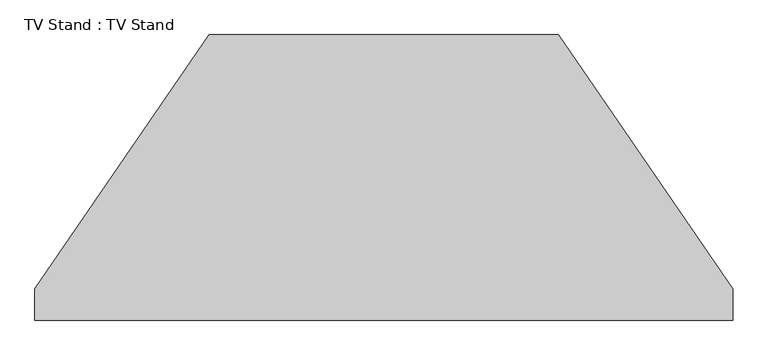
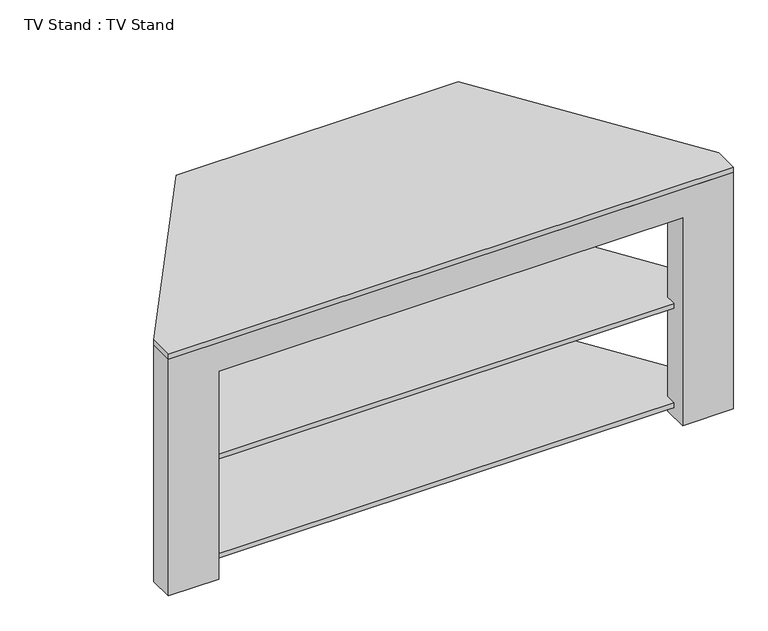
"""IFC4 building model written with IfcOpenShell, lengths in millimetres: furniture geometry, TV Stand : TV Stand."""

import ifcopenshell
import ifcopenshell.guid

model = None  # the IFC model being written
_history = None  # IfcOwnerHistory: only IFC2X3 demands one
_inside = {}  # id of a spatial element -> (the spatial element, [elements in it])
_under = {}  # id of a project, library or spatial element -> (it, [spatial elements below it])
_declared = {}  # id of a project -> (the project, [libraries it declares])
_typed = {}  # id of a type object -> (the type object, [elements of that type])
_made_of = {}  # id of a material, layer set ... -> (it, [elements and type objects made of it])


def new_model(schema):
    """Start an empty IFC model of exactly this schema.

    Asked for "IFC4X3", IfcOpenShell would pick the latest addendum, in which some entities
    have other attributes; the version numbers below select the first issue.
    IFC2X3 requires an IfcOwnerHistory on every rooted entity: one is made here for all.
    """
    global model, _history
    if schema == "IFC4X3":
        model = ifcopenshell.file(schema_version=(4, 3, 0, 0))
    else:
        model = ifcopenshell.file(schema=schema)
    _inside.clear()
    _under.clear()
    _declared.clear()
    _typed.clear()
    _made_of.clear()
    _history = None
    if model.schema == "IFC2X3":
        org = make("IfcOrganization", Name="unknown")
        user = make(
            "IfcPersonAndOrganization",
            ThePerson=make("IfcPerson", FamilyName="unknown"),
            TheOrganization=org,
        )
        app = make(
            "IfcApplication",
            ApplicationDeveloper=org,
            Version="unknown",
            ApplicationFullName="unknown",
            ApplicationIdentifier="unknown",
        )
        _history = make(
            "IfcOwnerHistory",
            OwningUser=user,
            OwningApplication=app,
            ChangeAction="ADDED",
            CreationDate=0,
        )
    return model


def make(cls, **values):
    """One entity of the class cls with the attributes given. An attribute that is None is left unset."""
    return model.create_entity(
        cls, **{name: value for name, value in values.items() if value is not None}
    )


def rooted(cls, **values):
    """An entity with a GlobalId (a new one), such as an element, a storey or a relation."""
    return make(cls, GlobalId=ifcopenshell.guid.new(), OwnerHistory=_history, **values)


def si_unit(unit_type, name, prefix=None):
    """IfcSIUnit, for example si_unit("LENGTHUNIT", "METRE", prefix="MILLI")."""
    return make("IfcSIUnit", UnitType=unit_type, Prefix=prefix, Name=name)


def assignment(units):
    """IfcUnitAssignment: the units of a project."""
    return None if units is None else make("IfcUnitAssignment", Units=units)


def point(xyz):
    """IfcCartesianPoint."""
    return None if xyz is None else make("IfcCartesianPoint", Coordinates=xyz)


def direction(xyz):
    """IfcDirection."""
    return None if xyz is None else make("IfcDirection", DirectionRatios=xyz)


def frame(location, z_axis=None, x_axis=None):
    """IfcAxis2Placement3D, a coordinate frame: its origin and axes. An axis left out is left unset."""
    return make(
        "IfcAxis2Placement3D",
        Location=point(location),
        Axis=direction(z_axis),
        RefDirection=direction(x_axis),
    )


def frame_2d(location, x_axis=None):
    """IfcAxis2Placement2D, a coordinate frame in the plane: its origin and x axis."""
    return make(
        "IfcAxis2Placement2D", Location=point(location), RefDirection=direction(x_axis)
    )


def origin():
    """The frame at (0, 0, 0) with its axes left unset."""
    return frame((0.0, 0.0, 0.0))


def place(relative_to, where):
    """IfcLocalPlacement: puts the frame where relative to a parent placement (None: the world)."""
    return make(
        "IfcLocalPlacement", PlacementRelTo=relative_to, RelativePlacement=where
    )


def context(
    kind, dimensions, precision=None, world=None, true_north=None, identifier=None
):
    """IfcGeometricRepresentationContext, for example the 3D "Model" context."""
    return make(
        "IfcGeometricRepresentationContext",
        ContextIdentifier=identifier,
        ContextType=kind,
        CoordinateSpaceDimension=dimensions,
        Precision=precision,
        WorldCoordinateSystem=world,
        TrueNorth=true_north,
    )


def project(units=None, contexts=None):
    """IfcProject with its units and contexts."""
    return rooted(
        "IfcProject",
        Name="project",
        RepresentationContexts=contexts,
        UnitsInContext=assignment(units),
    )


def spatial(cls, under=None, at=None, **own):
    """A site, building, storey or space (cls), placed at a placement, below another one or the project."""
    s = rooted(cls, ObjectPlacement=at, **own)
    if under is not None:
        _under.setdefault(under.id(), (under, []))[1].append(s)
    return s


def polyline(points):
    """IfcPolyline through the points."""
    return make("IfcPolyline", Points=[point(p) for p in points])


def circle_curve(where, radius):
    """IfcCircle in the frame where."""
    return make("IfcCircle", Position=where, Radius=radius)


def trimmed(basis, trim1, trim2, sense, master):
    """IfcTrimmedCurve: the piece of a basis curve between two trims."""
    return make(
        "IfcTrimmedCurve",
        BasisCurve=basis,
        Trim1=trim1,
        Trim2=trim2,
        SenseAgreement=sense,
        MasterRepresentation=master,
    )


def segment(curve, same_sense, transition):
    """IfcCompositeCurveSegment."""
    return make(
        "IfcCompositeCurveSegment",
        Transition=transition,
        SameSense=same_sense,
        ParentCurve=curve,
    )


def composite_curve(segments, self_intersect=None):
    """IfcCompositeCurve: segments joined end to end."""
    return make("IfcCompositeCurve", Segments=segments, SelfIntersect=self_intersect)


def outline(outer, holes=None, kind="AREA"):
    """IfcArbitraryClosedProfileDef: a profile drawn as a closed curve; with holes, ...WithVoids."""
    if holes is None:
        return make("IfcArbitraryClosedProfileDef", ProfileType=kind, OuterCurve=outer)
    return make(
        "IfcArbitraryProfileDefWithVoids",
        ProfileType=kind,
        OuterCurve=outer,
        InnerCurves=holes,
    )


def extrude(swept, where, along, depth):
    """IfcExtrudedAreaSolid: the profile swept, set in the frame where, extruded along a direction by depth."""
    return make(
        "IfcExtrudedAreaSolid",
        SweptArea=swept,
        Position=where,
        ExtrudedDirection=direction(along),
        Depth=depth,
    )


def faces_of(points, faces, orient=None, outer=None):
    """IfcFace entities. A face is a list of loops; a loop is a list of indices into points, from 0.

    orient and outer hold one flag for each loop. By default every Orientation is true, the
    first loop of a face is its IfcFaceOuterBound and the others are IfcFaceBound.
    """
    made = []
    for i, loops in enumerate(faces):
        bounds = []
        for j, loop in enumerate(loops):
            is_outer = j == 0 if outer is None else outer[i][j]
            bounds.append(
                make(
                    "IfcFaceOuterBound" if is_outer else "IfcFaceBound",
                    Bound=make("IfcPolyLoop", Polygon=[points[k] for k in loop]),
                    Orientation=True if orient is None else orient[i][j],
                )
            )
        made.append(make("IfcFace", Bounds=bounds))
    return made


def faceted_brep(points, faces, orient=None, outer=None, voids=None):
    """IfcFacetedBrep: a solid bounded by flat faces; with voids (closed shells), ...WithVoids."""
    shared = [point(p) for p in points]
    hull = make("IfcClosedShell", CfsFaces=faces_of(shared, faces, orient, outer))
    if voids is None:
        return make("IfcFacetedBrep", Outer=hull)
    return make(
        "IfcFacetedBrepWithVoids",
        Outer=hull,
        Voids=[
            make(cls, CfsFaces=faces_of(shared, fs, o, b)) for cls, fs, o, b in voids
        ],
    )


def shape(context_of_items, identifier, shape_type, items):
    """IfcShapeRepresentation: the items that make up one representation, for example the "Body"."""
    return make(
        "IfcShapeRepresentation",
        ContextOfItems=context_of_items,
        RepresentationIdentifier=identifier,
        RepresentationType=shape_type,
        Items=items,
    )


def source(mapping_origin, context_of_items, identifier, shape_type, items):
    """IfcRepresentationMap: a shape defined once, which mapped items show again and again."""
    return make(
        "IfcRepresentationMap",
        MappingOrigin=mapping_origin,
        MappedRepresentation=shape(context_of_items, identifier, shape_type, items),
    )


def transform(
    local_origin,
    x_axis=None,
    y_axis=None,
    z_axis=None,
    scale=None,
    scale2=None,
    scale3=None,
    uniform=True,
):
    """IfcCartesianTransformationOperator3D, or its non-uniform kind. x_axis, y_axis, z_axis: its Axis1, 2, 3."""
    if uniform:
        return make(
            "IfcCartesianTransformationOperator3D",
            Axis1=direction(x_axis),
            Axis2=direction(y_axis),
            LocalOrigin=point(local_origin),
            Scale=scale,
            Axis3=direction(z_axis),
        )
    return make(
        "IfcCartesianTransformationOperator3DnonUniform",
        Axis1=direction(x_axis),
        Axis2=direction(y_axis),
        LocalOrigin=point(local_origin),
        Scale=scale,
        Axis3=direction(z_axis),
        Scale2=scale2,
        Scale3=scale3,
    )


def mapped(mapping_source, mapping_target):
    """IfcMappedItem: shows the shape of a source again, moved by a transform."""
    return make(
        "IfcMappedItem", MappingSource=mapping_source, MappingTarget=mapping_target
    )


def made_of(thing, what):
    """Note that an element or type object is made of a material, layer set ...; save() writes the relation."""
    if what is not None:
        _made_of.setdefault(what.id(), (what, []))[1].append(thing)
    return thing


def element(
    cls,
    number,
    at=None,
    inside=None,
    cuts=None,
    type_object=None,
    material=None,
    context=None,
    identifier="Body",
    shape_type=None,
    held_by="IfcProductDefinitionShape",
    body=None,
    shapes=None,
    **own,
):
    """One element of the class cls, such as IfcWall. Its Tag is "e" and its number.

    at: its placement. inside: the storey or other place that contains it. cuts: it is an
    opening in that element (IfcRelVoidsElement). A single representation is given by context,
    identifier, shape_type and body (its items); several are given by shapes. held_by: the class
    of the entity that holds the representations. save() writes the other relations.
    """
    e = rooted(cls, Tag="e%d" % number, ObjectPlacement=at, **own)
    if body is not None:
        shapes = [shape(context, identifier, shape_type, body)]
    if shapes is not None:
        e.Representation = make(held_by, Representations=shapes)
    if inside is not None:
        _inside.setdefault(inside.id(), (inside, []))[1].append(e)
    if cuts is not None:
        rooted(
            "IfcRelVoidsElement", RelatingBuildingElement=cuts, RelatedOpeningElement=e
        )
    if type_object is not None:
        _typed.setdefault(type_object.id(), (type_object, []))[1].append(e)
    return made_of(e, material)


def aggregate(whole, parts):
    """IfcRelAggregates: a whole, such as a stair, and the parts it consists of."""
    return rooted("IfcRelAggregates", RelatingObject=whole, RelatedObjects=parts)


def save(model, path):
    """Write the relations noted so far, then the file.

    IfcRelAggregates (storeys below a building ...), IfcRelContainedInSpatialStructure (elements
    in a storey), IfcRelDefinesByType, IfcRelAssociatesMaterial and IfcRelDeclares: one each for
    every whole, place, type object, material and project.
    """
    for whole, parts in _under.values():
        aggregate(whole, parts)
    for where, things in _inside.values():
        rooted(
            "IfcRelContainedInSpatialStructure",
            RelatedElements=things,
            RelatingStructure=where,
        )
    for kind, things in _typed.values():
        rooted("IfcRelDefinesByType", RelatedObjects=things, RelatingType=kind)
    for what, things in _made_of.values():
        rooted("IfcRelAssociatesMaterial", RelatedObjects=things, RelatingMaterial=what)
    for by, libraries in _declared.values():
        rooted("IfcRelDeclares", RelatingContext=by, RelatedDefinitions=libraries)
    model.write(path)


def tv_stand_tv_stand_6ce107e5(model_context):
    return source(origin(), model_context, "Body", "SolidModel", [
        extrude(outline(polyline([(425.1724814, -30.0), (633.9880021, -334.3295634), (633.9880021, -427.2), (-383.6119979, -427.2), (-383.6119979, -334.3295634), (-174.7964773, -30.0), (425.1724814, -30.0)])), frame((0.0, 0.0, 20.0), z_axis=(0.0, 0.0, 1.0), x_axis=(1.0, 0.0, 0.0)), (0.0, 0.0, 1.0), 10.0),
        extrude(outline(polyline([(425.1724814, -30.0), (633.9880021, -334.3295634), (633.9880021, -427.2), (-383.6119979, -427.2), (-383.6119979, -334.3295634), (-174.7964773, -30.0), (425.1724814, -30.0)])), frame((0.0, 0.0, 227.65), z_axis=(0.0, 0.0, 1.0), x_axis=(1.0, 0.0, 0.0)), (0.0, 0.0, 1.0), 10.0),
        extrude(outline(polyline([(404.5880021, 0.0), (683.9880021, -407.2), (683.9880021, -457.2), (-433.6119979, -457.2), (-433.6119979, -407.2), (-154.2119979, 0.0), (404.5880021, 0.0)])), frame((0.0, 0.0, 495.3), z_axis=(0.0, 0.0, 1.0), x_axis=(1.0, 0.0, 0.0)), (0.0, 0.0, 1.0), 10.0),
        extrude(outline(polyline([(-50.0, 495.3), (0.0, 495.3), (0.0, 0.0), (-50.0, 0.0), (-50.0, 20.0), (-30.0, 20.0), (-30.0, 30.0), (-50.0, 30.0), (-50.0, 227.65), (-30.0, 227.65), (-30.0, 237.65), (-50.0, 237.65), (-50.0, 495.3)])), frame((-154.2119979, 0.0, 0.0), z_axis=(1.0, 0.0, 0.0), x_axis=(0.0, 1.0, 0.0)), (0.0, 0.0, 1.0), 100.0),
        extrude(outline(polyline([(-50.0, 495.3), (0.0, 495.3), (0.0, 0.0), (-50.0, 0.0), (-50.0, 20.0), (-30.0, 20.0), (-30.0, 30.0), (-50.0, 30.0), (-50.0, 227.65), (-30.0, 227.65), (-30.0, 237.65), (-50.0, 237.65), (-50.0, 495.3)])), frame((304.5880021, 0.0, 0.0), z_axis=(1.0, 0.0, 0.0), x_axis=(0.0, 1.0, 0.0)), (0.0, 0.0, 1.0), 100.0),
        faceted_brep([(-433.6119979, -457.2, 0.0), (-333.6119979, -457.2, 0.0), (-333.6119979, -457.2, 435.3), (583.9880021, -457.2, 435.3), (583.9880021, -457.2, 0.0), (683.9880021, -457.2, 0.0), (683.9880021, -457.2, 495.3), (-433.6119979, -457.2, 495.3), (-433.6119979, -407.2, 0.0), (-433.6119979, -407.2, 495.3), (683.9880021, -407.2, 495.3), (683.9880021, -407.2, 0.0), (583.9880021, -407.2, 0.0), (583.9880021, -407.2, 20.0), (633.9880021, -407.2, 20.0), (633.9880021, -407.2, 30.0), (583.9880021, -407.2, 30.0), (583.9880021, -407.2, 227.65), (633.9880021, -407.2, 227.65), (633.9880021, -407.2, 237.65), (583.9880021, -407.2, 237.65), (583.9880021, -407.2, 435.3), (-333.6119979, -407.2, 435.3), (-333.6119979, -407.2, 237.65), (-383.6119979, -407.2, 237.65), (-383.6119979, -407.2, 227.65), (-333.6119979, -407.2, 227.65), (-333.6119979, -407.2, 30.0), (-383.6119979, -407.2, 30.0), (-383.6119979, -407.2, 20.0), (-333.6119979, -407.2, 20.0), (-333.6119979, -407.2, 0.0), (-333.6119979, -427.2, 20.0), (-333.6119979, -427.2, 30.0), (-333.6119979, -427.2, 227.65), (-333.6119979, -427.2, 237.65), (583.9880021, -427.2, 237.65), (583.9880021, -427.2, 227.65), (583.9880021, -427.2, 30.0), (583.9880021, -427.2, 20.0), (633.9880021, -427.2, 237.65), (-383.6119979, -427.2, 237.65), (-383.6119979, -427.2, 227.65), (633.9880021, -427.2, 227.65), (633.9880021, -427.2, 30.0), (-383.6119979, -427.2, 30.0), (-383.6119979, -427.2, 20.0), (633.9880021, -427.2, 20.0)], [[[0, 1, 2, 3, 4, 5, 6, 7]], [[8, 9, 10, 11, 12, 13, 14, 15, 16, 17, 18, 19, 20, 21, 22, 23, 24, 25, 26, 27, 28, 29, 30, 31]], [[1, 0, 8, 31]], [[2, 1, 31, 30, 32, 33, 27, 26, 34, 35, 23, 22]], [[3, 2, 22, 21]], [[4, 3, 21, 20, 36, 37, 17, 16, 38, 39, 13, 12]], [[5, 4, 12, 11]], [[6, 5, 11, 10]], [[7, 6, 10, 9]], [[0, 7, 9, 8]], [[19, 40, 36, 20]], [[35, 41, 24, 23]], [[25, 42, 34, 26]], [[37, 43, 18, 17]], [[41, 42, 25, 24]], [[42, 41, 35, 34]], [[40, 43, 37, 36]], [[43, 40, 19, 18]], [[15, 44, 38, 16]], [[33, 45, 28, 27]], [[29, 46, 32, 30]], [[39, 47, 14, 13]], [[45, 46, 29, 28]], [[46, 45, 33, 32]], [[44, 47, 39, 38]], [[47, 44, 15, 14]]]),
        extrude(outline(polyline([(0.0, 304.5880021), (495.3, 304.5880021), (495.3, -54.2119979), (0.0, -54.2119979), (0.0, 304.5880021)]), holes=[composite_curve([segment(polyline([(242.65, 145.1700818), (242.65, 105.2059224)]), True, "CONTINUOUS"), segment(trimmed(circle_curve(frame_2d((255.15, 105.2059224)), 12.5), [point((242.65, 105.2059224))], [point((267.65, 105.2059224))], True, "CARTESIAN"), True, "CONTINUOUS"), segment(polyline([(267.65, 105.2059224), (267.65, 145.1700818)]), True, "CONTINUOUS"), segment(trimmed(circle_curve(frame_2d((255.15, 145.1700818)), 12.5), [point((267.65, 145.1700818))], [point((242.65, 145.1700818))], True, "CARTESIAN"), True, "CONTINUOUS")], self_intersect=False), composite_curve([segment(polyline([(35.0, 145.1880021), (35.0, 105.2059224)]), True, "CONTINUOUS"), segment(trimmed(circle_curve(frame_2d((47.5, 105.2059224)), 12.5), [point((35.0, 105.2059224))], [point((60.0, 105.2059224))], True, "CARTESIAN"), True, "CONTINUOUS"), segment(polyline([(60.0, 105.2059224), (60.0, 145.1880021)]), True, "CONTINUOUS"), segment(trimmed(circle_curve(frame_2d((47.5, 145.1880021)), 12.5), [point((60.0, 145.1880021))], [point((35.0, 145.1880021))], True, "CARTESIAN"), True, "CONTINUOUS")], self_intersect=False)]), frame((0.0, -30.0, 0.0), z_axis=(0.0, 1.0, 0.0), x_axis=(0.0, 0.0, 1.0)), (0.0, 0.0, 1.0), 10.0),
    ])


if __name__ == "__main__":
    model = new_model("IFC4")
    model_context = context("Model", 3, world=origin())
    ifc_project = project(units=[si_unit("LENGTHUNIT", "METRE", prefix="MILLI")], contexts=[model_context])
    site = spatial("IfcSite", under=ifc_project)
    building = spatial("IfcBuilding", under=site)
    placement = place(None, origin())
    tv_stand_tv_stand_shape = tv_stand_tv_stand_6ce107e5(model_context)
    element("IfcFurniture", 1, ObjectType="TV Stand : TV Stand", at=placement, inside=building, context=model_context, shape_type="MappedRepresentation", body=[
        mapped(tv_stand_tv_stand_shape, transform((0.0, 0.0, 0.0), x_axis=(1.0, 0.0, 0.0), y_axis=(0.0, 1.0, 0.0), z_axis=(0.0, 0.0, 1.0))),
    ])
    save(model, "model.ifc")

# Revit data of these elements
# Type "TV Stand : TV Stand"
#   Depth = 1' - 6"
#   Width = 3' - 8"
#   Height = 1' - 7 1/2"
#   Finish = Melamine - Gray
# Element 1 (IfcFurniture, "TV Stand : TV Stand")
#   Materials on its faces: "Melamine - Gray", "Glass - Shelves"
# Materials
#   "Melamine - Gray": class "Wood", colour RGB 49 49 49, transparency 0
#   "Glass - Shelves": class "Glass", colour RGB 167 167 167, transparency 0.9
